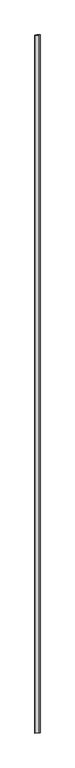
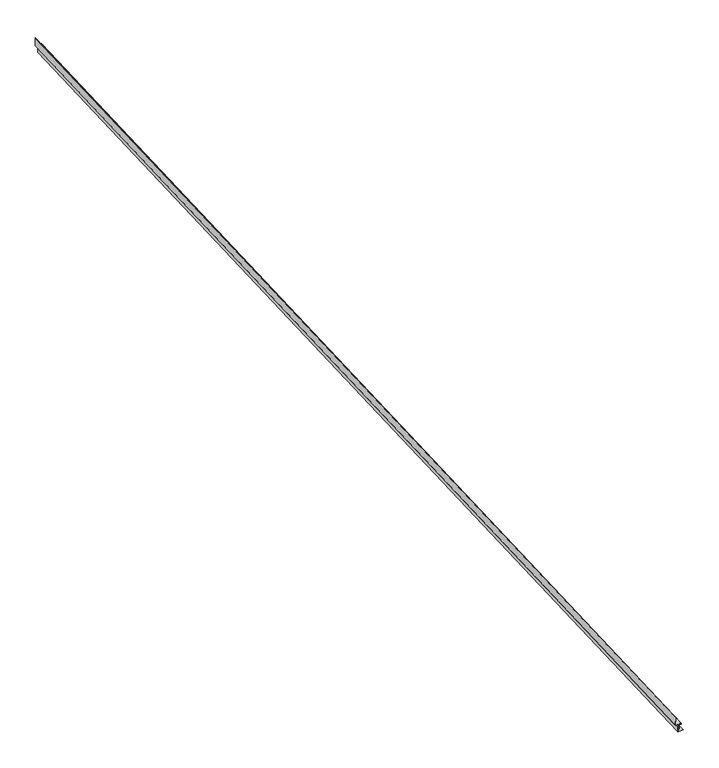
"""IFC4 building model written with IfcOpenShell, lengths in millimetres: proxy geometry, Generic Models 2:Generic Models 2:310765:Generic Models 2:310765 : Generic Models 2:Generic Models 2:310765:199 : Generic Models 2:Generic Models 2:310765:Generic Models 2:310765 : Generic Models 2:Generic Models 2:310765:300385."""

import ifcopenshell
import ifcopenshell.guid

model = None  # the IFC model being written
_history = None  # IfcOwnerHistory: only IFC2X3 demands one
_inside = {}  # id of a spatial element -> (the spatial element, [elements in it])
_under = {}  # id of a project, library or spatial element -> (it, [spatial elements below it])
_declared = {}  # id of a project -> (the project, [libraries it declares])
_typed = {}  # id of a type object -> (the type object, [elements of that type])
_made_of = {}  # id of a material, layer set ... -> (it, [elements and type objects made of it])


def new_model(schema):
    """Start an empty IFC model of exactly this schema.

    Asked for "IFC4X3", IfcOpenShell would pick the latest addendum, in which some entities
    have other attributes; the version numbers below select the first issue.
    IFC2X3 requires an IfcOwnerHistory on every rooted entity: one is made here for all.
    """
    global model, _history
    if schema == "IFC4X3":
        model = ifcopenshell.file(schema_version=(4, 3, 0, 0))
    else:
        model = ifcopenshell.file(schema=schema)
    _inside.clear()
    _under.clear()
    _declared.clear()
    _typed.clear()
    _made_of.clear()
    _history = None
    if model.schema == "IFC2X3":
        org = make("IfcOrganization", Name="unknown")
        user = make(
            "IfcPersonAndOrganization",
            ThePerson=make("IfcPerson", FamilyName="unknown"),
            TheOrganization=org,
        )
        app = make(
            "IfcApplication",
            ApplicationDeveloper=org,
            Version="unknown",
            ApplicationFullName="unknown",
            ApplicationIdentifier="unknown",
        )
        _history = make(
            "IfcOwnerHistory",
            OwningUser=user,
            OwningApplication=app,
            ChangeAction="ADDED",
            CreationDate=0,
        )
    return model


def make(cls, **values):
    """One entity of the class cls with the attributes given. An attribute that is None is left unset."""
    return model.create_entity(
        cls, **{name: value for name, value in values.items() if value is not None}
    )


def rooted(cls, **values):
    """An entity with a GlobalId (a new one), such as an element, a storey or a relation."""
    return make(cls, GlobalId=ifcopenshell.guid.new(), OwnerHistory=_history, **values)


def si_unit(unit_type, name, prefix=None):
    """IfcSIUnit, for example si_unit("LENGTHUNIT", "METRE", prefix="MILLI")."""
    return make("IfcSIUnit", UnitType=unit_type, Prefix=prefix, Name=name)


def assignment(units):
    """IfcUnitAssignment: the units of a project."""
    return None if units is None else make("IfcUnitAssignment", Units=units)


def point(xyz):
    """IfcCartesianPoint."""
    return None if xyz is None else make("IfcCartesianPoint", Coordinates=xyz)


def direction(xyz):
    """IfcDirection."""
    return None if xyz is None else make("IfcDirection", DirectionRatios=xyz)


def frame(location, z_axis=None, x_axis=None):
    """IfcAxis2Placement3D, a coordinate frame: its origin and axes. An axis left out is left unset."""
    return make(
        "IfcAxis2Placement3D",
        Location=point(location),
        Axis=direction(z_axis),
        RefDirection=direction(x_axis),
    )


def origin():
    """The frame at (0, 0, 0) with its axes left unset."""
    return frame((0.0, 0.0, 0.0))


def place(relative_to, where):
    """IfcLocalPlacement: puts the frame where relative to a parent placement (None: the world)."""
    return make(
        "IfcLocalPlacement", PlacementRelTo=relative_to, RelativePlacement=where
    )


def context(
    kind, dimensions, precision=None, world=None, true_north=None, identifier=None
):
    """IfcGeometricRepresentationContext, for example the 3D "Model" context."""
    return make(
        "IfcGeometricRepresentationContext",
        ContextIdentifier=identifier,
        ContextType=kind,
        CoordinateSpaceDimension=dimensions,
        Precision=precision,
        WorldCoordinateSystem=world,
        TrueNorth=true_north,
    )


def project(units=None, contexts=None):
    """IfcProject with its units and contexts."""
    return rooted(
        "IfcProject",
        Name="project",
        RepresentationContexts=contexts,
        UnitsInContext=assignment(units),
    )


def spatial(cls, under=None, at=None, **own):
    """A site, building, storey or space (cls), placed at a placement, below another one or the project."""
    s = rooted(cls, ObjectPlacement=at, **own)
    if under is not None:
        _under.setdefault(under.id(), (under, []))[1].append(s)
    return s


def polyline(points):
    """IfcPolyline through the points."""
    return make("IfcPolyline", Points=[point(p) for p in points])


def outline(outer, holes=None, kind="AREA"):
    """IfcArbitraryClosedProfileDef: a profile drawn as a closed curve; with holes, ...WithVoids."""
    if holes is None:
        return make("IfcArbitraryClosedProfileDef", ProfileType=kind, OuterCurve=outer)
    return make(
        "IfcArbitraryProfileDefWithVoids",
        ProfileType=kind,
        OuterCurve=outer,
        InnerCurves=holes,
    )


def extrude(swept, where, along, depth):
    """IfcExtrudedAreaSolid: the profile swept, set in the frame where, extruded along a direction by depth."""
    return make(
        "IfcExtrudedAreaSolid",
        SweptArea=swept,
        Position=where,
        ExtrudedDirection=direction(along),
        Depth=depth,
    )


def shape(context_of_items, identifier, shape_type, items):
    """IfcShapeRepresentation: the items that make up one representation, for example the "Body"."""
    return make(
        "IfcShapeRepresentation",
        ContextOfItems=context_of_items,
        RepresentationIdentifier=identifier,
        RepresentationType=shape_type,
        Items=items,
    )


def source(mapping_origin, context_of_items, identifier, shape_type, items):
    """IfcRepresentationMap: a shape defined once, which mapped items show again and again."""
    return make(
        "IfcRepresentationMap",
        MappingOrigin=mapping_origin,
        MappedRepresentation=shape(context_of_items, identifier, shape_type, items),
    )


def transform(
    local_origin,
    x_axis=None,
    y_axis=None,
    z_axis=None,
    scale=None,
    scale2=None,
    scale3=None,
    uniform=True,
):
    """IfcCartesianTransformationOperator3D, or its non-uniform kind. x_axis, y_axis, z_axis: its Axis1, 2, 3."""
    if uniform:
        return make(
            "IfcCartesianTransformationOperator3D",
            Axis1=direction(x_axis),
            Axis2=direction(y_axis),
            LocalOrigin=point(local_origin),
            Scale=scale,
            Axis3=direction(z_axis),
        )
    return make(
        "IfcCartesianTransformationOperator3DnonUniform",
        Axis1=direction(x_axis),
        Axis2=direction(y_axis),
        LocalOrigin=point(local_origin),
        Scale=scale,
        Axis3=direction(z_axis),
        Scale2=scale2,
        Scale3=scale3,
    )


def mapped(mapping_source, mapping_target):
    """IfcMappedItem: shows the shape of a source again, moved by a transform."""
    return make(
        "IfcMappedItem", MappingSource=mapping_source, MappingTarget=mapping_target
    )


def made_of(thing, what):
    """Note that an element or type object is made of a material, layer set ...; save() writes the relation."""
    if what is not None:
        _made_of.setdefault(what.id(), (what, []))[1].append(thing)
    return thing


def element(
    cls,
    number,
    at=None,
    inside=None,
    cuts=None,
    type_object=None,
    material=None,
    context=None,
    identifier="Body",
    shape_type=None,
    held_by="IfcProductDefinitionShape",
    body=None,
    shapes=None,
    **own,
):
    """One element of the class cls, such as IfcWall. Its Tag is "e" and its number.

    at: its placement. inside: the storey or other place that contains it. cuts: it is an
    opening in that element (IfcRelVoidsElement). A single representation is given by context,
    identifier, shape_type and body (its items); several are given by shapes. held_by: the class
    of the entity that holds the representations. save() writes the other relations.
    """
    e = rooted(cls, Tag="e%d" % number, ObjectPlacement=at, **own)
    if body is not None:
        shapes = [shape(context, identifier, shape_type, body)]
    if shapes is not None:
        e.Representation = make(held_by, Representations=shapes)
    if inside is not None:
        _inside.setdefault(inside.id(), (inside, []))[1].append(e)
    if cuts is not None:
        rooted(
            "IfcRelVoidsElement", RelatingBuildingElement=cuts, RelatedOpeningElement=e
        )
    if type_object is not None:
        _typed.setdefault(type_object.id(), (type_object, []))[1].append(e)
    return made_of(e, material)


def aggregate(whole, parts):
    """IfcRelAggregates: a whole, such as a stair, and the parts it consists of."""
    return rooted("IfcRelAggregates", RelatingObject=whole, RelatedObjects=parts)


def save(model, path):
    """Write the relations noted so far, then the file.

    IfcRelAggregates (storeys below a building ...), IfcRelContainedInSpatialStructure (elements
    in a storey), IfcRelDefinesByType, IfcRelAssociatesMaterial and IfcRelDeclares: one each for
    every whole, place, type object, material and project.
    """
    for whole, parts in _under.values():
        aggregate(whole, parts)
    for where, things in _inside.values():
        rooted(
            "IfcRelContainedInSpatialStructure",
            RelatedElements=things,
            RelatingStructure=where,
        )
    for kind, things in _typed.values():
        rooted("IfcRelDefinesByType", RelatedObjects=things, RelatingType=kind)
    for what, things in _made_of.values():
        rooted("IfcRelAssociatesMaterial", RelatedObjects=things, RelatingMaterial=what)
    for by, libraries in _declared.values():
        rooted("IfcRelDeclares", RelatingContext=by, RelatedDefinitions=libraries)
    model.write(path)


def generic_models_8f1aa049(model_context):
    return source(origin(), model_context, "Body", "SweptSolid", [
        extrude(outline(polyline([(146.0500001, 0.0), (146.0500001, -64.1575641), (155.5750001, -64.1575641), (155.5750001, -46.6950641), (157.1625, -46.6950641), (157.1625, -65.7450641), (144.4625, -65.7450641), (144.4625, -1.5875), (55.5625, -1.5875), (55.5625, 0.0), (146.0500001, 0.0)])), frame((579320.4117239, -579018.008545, 4181.1618628), z_axis=(0.0, 0.9991330730923567, 0.041630544712067834), x_axis=(0.0, 0.041630544712067834, -0.9991330730923567)), (0.0, 0.0, 1.0), 12335.2906118),
        extrude(outline(polyline([(151.60625, -42.3509311), (151.60625, -61.2200628), (150.01875, -61.2200628), (150.01875, -40.7634311), (202.40625, -40.7634311), (202.40625, -42.3509311), (151.60625, -42.3509311)])), frame((579320.4117239, -579018.008545, 4181.1618628), z_axis=(0.0, 0.9991330730923567, 0.041630544712067834), x_axis=(0.0, 0.041630544712067834, -0.9991330730923567)), (0.0, 0.0, 1.0), 12335.2906118),
        extrude(outline(polyline([(235.74375, -30.1625), (235.74375, -91.3825628), (234.1562501, -91.3825628), (234.1562501, -31.75), (172.24375, -31.75), (172.24375, -30.1625), (235.74375, -30.1625)])), frame((579320.4117239, -579018.008545, 4181.1618628), z_axis=(0.0, 0.9991330730923567, 0.041630544712067834), x_axis=(0.0, 0.041630544712067834, -0.9991330730923567)), (0.0, 0.0, 1.0), 12335.2906118),
    ])


if __name__ == "__main__":
    model = new_model("IFC4")
    model_context = context("Model", 3, world=origin())
    ifc_project = project(units=[si_unit("LENGTHUNIT", "METRE", prefix="MILLI")], contexts=[model_context])
    site = spatial("IfcSite", under=ifc_project)
    building = spatial("IfcBuilding", under=site)
    placement = place(None, origin())
    generic_models_shape = generic_models_8f1aa049(model_context)
    element("IfcBuildingElementProxy", 1, Name="Generic Models 2:Generic Models 2:310765:Generic Models 2:310765 : Generic Models 2:Generic Models 2:310765:199 : Generic Models 2:Generic Models 2:310765:Generic Models 2:310765 : Generic Models 2:Generic Models 2:310765:300385", ObjectType="Generic Models 2:Generic Models 2:310765:Generic Models 2:310765 : Generic Models 2:Generic Models 2:310765:199 : Generic Models 2:Generic Models 2:310765:Generic Models 2:310765 : Generic Models 2:Generic Models 2:310765:300385", at=placement, inside=building, context=model_context, shape_type="MappedRepresentation", body=[
        mapped(generic_models_shape, transform((0.0, 0.0, 0.0), x_axis=(1.0, 0.0, 0.0), y_axis=(0.0, 1.0, 0.0), z_axis=(0.0, 0.0, 1.0))),
    ])
    save(model, "model.ifc")

# Revit data of these elements
# Type "Generic Models 2:Generic Models 2:310765:Generic Models 2:310765 : Generic Models 2:Generic Models 2:310765:199 : Generic Models 2:Generic Models 2:310765:Generic Models 2:310765 : Generic Models 2:Generic Models 2:310765:300385"
#   NameOverride = "Generic Models 2:Generic Models 2:310765:Generic Models 2:310765 : Generic Models 2:Generic Models 2:310765:300385"
#   ObjectTypeOverride = "Generic Models 2:310765 : Generic Models 2:Generic Models 2:310765"
#   Reference = "Generic Models 2"
#   Tag = "300385"
# Element 1 (IfcBuildingElementProxy, "Generic Models 2:Generic Models 2:310765:Generic Models 2:310765 : Generic Models 2:Generic Models 2:310765:199 : Generic Models 2:Generic Models 2:310765:Generic Models 2:310765 : Generic Models 2:Generic Models 2:310765:300385")
#   Materials on its faces: "BRAKE METAL COUNTERFLASHING"
# Materials
#   "BRAKE METAL COUNTERFLASHING": class "Unassigned", colour RGB 182 182 182, transparency 0, Cost = 0
